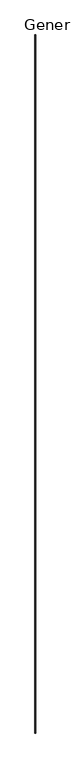
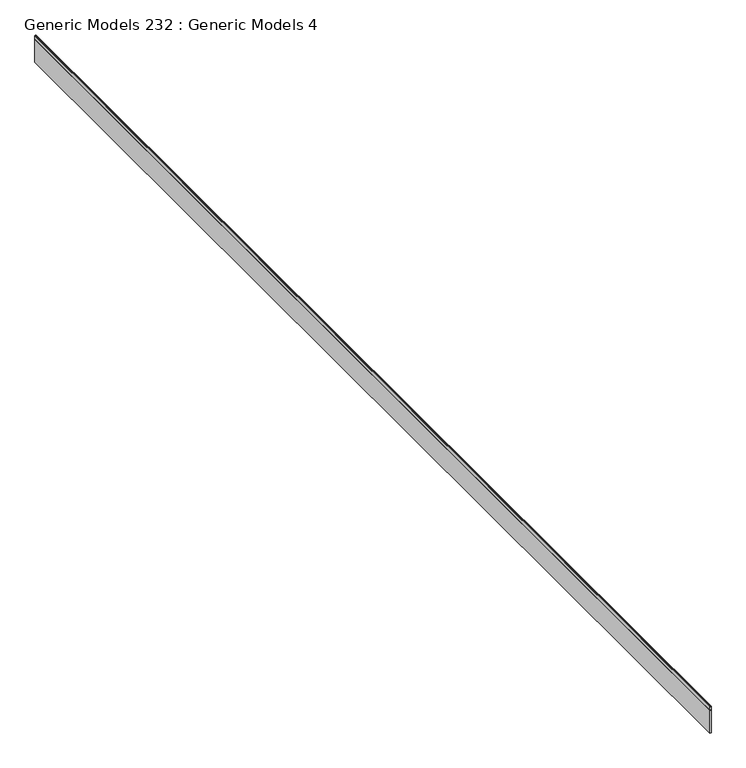
"""IFC4 building model written with IfcOpenShell, lengths in millimetres: proxy geometry, Generic Models 232 : Generic Models 4."""

from ifc_helpers import new_model, si_unit, frame, origin, place, context, project, spatial, polyline, outline, extrude, source, transform, mapped, element, save


def generic_models_232_generic_models_4_165a008c(model_context):
    return source(origin(), model_context, "Body", "SweptSolid", [
        extrude(outline(polyline([(126631.2488454, 1653.1175572), (126631.2488454, 1658.3748879), (126639.0636788, 1658.3748879), (126639.0636788, 1666.7475941), (126631.2488454, 1666.7475941), (126631.2488454, 1672.1675572), (126692.4566677, 1672.1675572), (126692.4566677, 1665.8175572), (126701.7355159, 1665.8175572), (126701.7355159, 1659.4675572), (126692.4566677, 1659.4675572), (126692.4566677, 1653.1175572), (126631.2488454, 1653.1175572)])), frame((0.0, -6864.9230338, 0.0), z_axis=(0.0, 1.0, 0.0), x_axis=(0.0, 0.0, 1.0)), (0.0, 0.0, 1.0), 18643.6),
        extrude(outline(polyline([(1672.1675572, -6864.9230338), (1653.1175572, -6864.9230338), (1653.1175572, 11778.6769662), (1672.1675572, 11778.6769662), (1672.1675572, -6864.9230338)])), frame((0.0, 0.0, 126250.2488454), z_axis=(0.0, 0.0, 1.0), x_axis=(1.0, 0.0, 0.0)), (0.0, 0.0, 1.0), 384.6166708),
    ])


if __name__ == "__main__":
    model = new_model("IFC4")
    model_context = context("Model", 3, world=origin())
    ifc_project = project(units=[si_unit("LENGTHUNIT", "METRE", prefix="MILLI")], contexts=[model_context])
    site = spatial("IfcSite", under=ifc_project)
    building = spatial("IfcBuilding", under=site)
    placement = place(None, origin())
    generic_models_232_generic_models_4_shape = generic_models_232_generic_models_4_165a008c(model_context)
    element("IfcBuildingElementProxy", 1, Name="Generic Models 232 : Generic Models 4", ObjectType="Generic Models 232 : Generic Models 4", at=placement, inside=building, context=model_context, shape_type="MappedRepresentation", body=[
        mapped(generic_models_232_generic_models_4_shape, transform((0.0, 0.0, 0.0), x_axis=(1.0, 0.0, 0.0), y_axis=(0.0, 1.0, 0.0), z_axis=(0.0, 0.0, 1.0))),
    ])
    save(model, "model.ifc")

# Revit data of these elements
# Element 1 (IfcBuildingElementProxy, "Generic Models 232 : Generic Models 4")
#   Materials on its faces: "_FIRE RETARDANT WOOD SIDING T.B.D"
# Materials
#   "_FIRE RETARDANT WOOD SIDING T.B.D": class "Generic", colour RGB 177 130 114, transparency 0, Cost = 0
